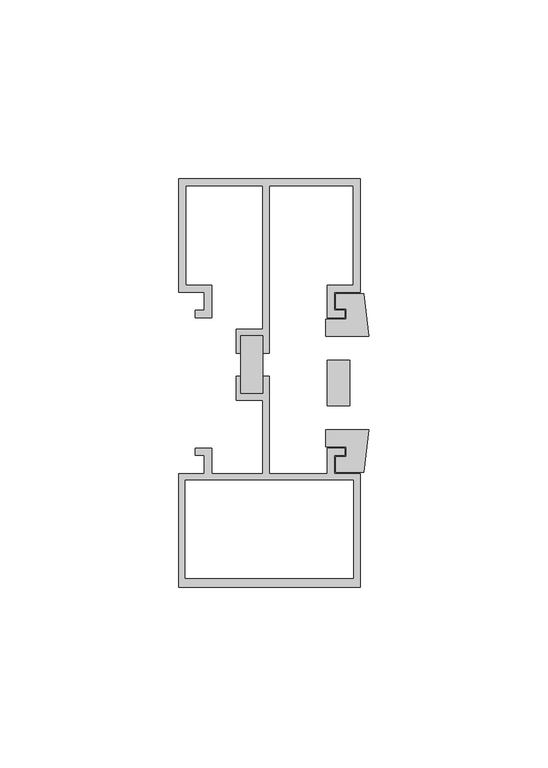
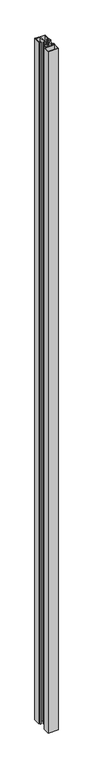
"""IFC4 building model written with IfcOpenShell, lengths in millimetres: proxy geometry, Generic Models 3:Generic Models 1:5:Generic Models 1:5 : Generic Models 3:Generic Models 1:300625:345888:Generic Models 1:5:Generic Models 1:5 : Generic Models 3:Generic Models 1:300625:345888 : Generic Models 3:Generic Models 1:5:Generic Models 1:5 : Generic Models 3:Generic Models 1:300625:345888:5 : Generic Models 3:Generic Models 1:5:Generic Models 1:5 : Generic Models 3:Generic Models 1:300625:345888:Generic Models 1:5:Generic Models 1:5 : Generic Models 3:Generic Models 1:300625:345888 : Generic Models 3:Generic Models 1:5:Generic Models 1:5 : Generic Models 3:Generic Models 1:300625:345888:301574."""

from ifc_helpers import new_model, si_unit, frame, origin, place, context, project, spatial, polyline, outline, extrude, source, transform, mapped, element, save


def generic_models_8cb2473c(model_context):
    return source(origin(), model_context, "Body", "SweptSolid", [
        extrude(outline(polyline([(592785.2574021, -579063.9802804), (592779.1776149, -579063.9802804), (592779.1776149, -579047.8688442), (592785.2574021, -579047.8688442), (592785.2574021, -579063.9802804)])), frame((0.0, 0.0, 66.3122056), z_axis=(0.0, 0.0, 1.0), x_axis=(1.0, 0.0, 0.0)), (0.0, 0.0, 1.0), 3584.971571),
        extrude(outline(polyline([(592809.6883176, -579067.3663841), (592803.3447692, -579067.3663841), (592803.3447692, -579054.6663841), (592809.6883176, -579054.6663841), (592809.6883176, -579067.3663841)])), frame((0.0, 0.0, 66.3122056), z_axis=(0.0, 0.0, 1.0), x_axis=(1.0, 0.0, 0.0)), (0.0, 0.0, 1.0), 3584.971571),
        extrude(outline(polyline([(592808.6614348, -579078.8588708), (592802.9478941, -579078.8588708), (592802.9478941, -579074.1048149), (592815.0181513, -579074.1048149), (592813.5572844, -579086.0026208), (592805.717575, -579086.0026208), (592805.717575, -579081.704549), (592808.6614348, -579081.704549), (592808.6614348, -579078.8588708)])), frame((0.0, 0.0, 66.3122056), z_axis=(0.0, 0.0, 1.0), x_axis=(1.0, 0.0, 0.0)), (0.0, 0.0, 1.0), 3584.971571),
        extrude(outline(polyline([(592813.5572844, -579036.0301474), (592815.0181513, -579047.9279532), (592802.9478941, -579047.9279532), (592802.9478941, -579043.1738974), (592808.6614348, -579043.1738974), (592808.6614348, -579040.3282192), (592805.717575, -579040.3282192), (592805.717575, -579036.0301474), (592813.5572844, -579036.0301474)])), frame((0.0, 0.0, 66.3122056), z_axis=(0.0, 0.0, 1.0), x_axis=(1.0, 0.0, 0.0)), (0.0, 0.0, 1.0), 3584.9377944),
        extrude(outline(polyline([(592761.7742239, -579118.1663841), (592761.7742239, -579086.3994958), (592768.9939713, -579086.3994958), (592768.9939713, -579081.307674), (592766.4747398, -579081.307674), (592766.4747398, -579079.2557458), (592771.0458995, -579079.2557458), (592771.0458995, -579086.3994958), (592785.2574021, -579086.3994958), (592785.2574021, -579065.8802139), (592777.8856601, -579065.8802139), (592777.8856601, -579059.1164506), (592779.1776149, -579059.1164506), (592779.1776149, -579063.9802804), (592785.2574021, -579063.9802804), (592785.2574021, -579059.1164506), (592787.1573356, -579059.1164506), (592787.1573356, -579086.3994958), (592803.3447691, -579086.3994958), (592803.3447691, -579079.2557458), (592808.2645598, -579079.2557458), (592808.2645598, -579081.307674), (592805.3207, -579081.307674), (592805.3207, -579086.3994958), (592812.5404473, -579086.3994958), (592812.5404473, -579118.1663841), (592761.7742239, -579118.1663841)]), holes=[polyline([(592810.6405138, -579088.2994293), (592763.6741574, -579088.2994293), (592763.6741574, -579115.6584719), (592810.6405138, -579115.6584719), (592810.6405138, -579088.2994293)])]), frame((0.0, 0.0, 66.3122056), z_axis=(0.0, 0.0, 1.0), x_axis=(1.0, 0.0, 0.0)), (0.0, 0.0, 1.0), 3584.971571),
        extrude(outline(polyline([(592808.2645598, -579040.7250942), (592808.2645598, -579042.7770224), (592803.3447691, -579042.7770224), (592803.3447691, -579033.7333389), (592810.6306483, -579033.7333389), (592810.6306483, -579005.8423149), (592787.1573356, -579005.8423149), (592787.1573356, -579052.732674), (592785.2574021, -579052.732674), (592785.2574021, -579047.8688442), (592779.1776149, -579047.8688442), (592779.1776149, -579052.732674), (592777.8856601, -579052.732674), (592777.8856601, -579045.9689107), (592785.2574021, -579045.9689107), (592785.2574021, -579005.8423149), (592763.6964365, -579005.8423149), (592763.6964365, -579033.7333389), (592771.0458995, -579033.7333389), (592771.0458995, -579042.7770224), (592766.4747398, -579042.7770224), (592766.4747398, -579040.7250942), (592768.9939713, -579040.7250942), (592768.9939713, -579035.6332724), (592761.7742239, -579035.6332724), (592761.7742239, -579003.8663841), (592812.5404473, -579003.8663841), (592812.5404473, -579035.6332724), (592805.3207, -579035.6332724), (592805.3207, -579040.7250942), (592808.2645598, -579040.7250942)])), frame((0.0, 0.0, 66.3122056), z_axis=(0.0, 0.0, 1.0), x_axis=(1.0, 0.0, 0.0)), (0.0, 0.0, 1.0), 3584.971571),
    ])


if __name__ == "__main__":
    model = new_model("IFC4")
    model_context = context("Model", 3, world=origin())
    ifc_project = project(units=[si_unit("LENGTHUNIT", "METRE", prefix="MILLI")], contexts=[model_context])
    site = spatial("IfcSite", under=ifc_project)
    building = spatial("IfcBuilding", under=site)
    placement = place(None, origin())
    generic_models_shape = generic_models_8cb2473c(model_context)
    element("IfcBuildingElementProxy", 1, Name="Generic Models 3:Generic Models 1:5:Generic Models 1:5 : Generic Models 3:Generic Models 1:300625:345888:Generic Models 1:5:Generic Models 1:5 : Generic Models 3:Generic Models 1:300625:345888 : Generic Models 3:Generic Models 1:5:Generic Models 1:5 : Generic Models 3:Generic Models 1:300625:345888:5 : Generic Models 3:Generic Models 1:5:Generic Models 1:5 : Generic Models 3:Generic Models 1:300625:345888:Generic Models 1:5:Generic Models 1:5 : Generic Models 3:Generic Models 1:300625:345888 : Generic Models 3:Generic Models 1:5:Generic Models 1:5 : Generic Models 3:Generic Models 1:300625:345888:301574", ObjectType="Generic Models 3:Generic Models 1:5:Generic Models 1:5 : Generic Models 3:Generic Models 1:300625:345888:Generic Models 1:5:Generic Models 1:5 : Generic Models 3:Generic Models 1:300625:345888 : Generic Models 3:Generic Models 1:5:Generic Models 1:5 : Generic Models 3:Generic Models 1:300625:345888:5 : Generic Models 3:Generic Models 1:5:Generic Models 1:5 : Generic Models 3:Generic Models 1:300625:345888:Generic Models 1:5:Generic Models 1:5 : Generic Models 3:Generic Models 1:300625:345888 : Generic Models 3:Generic Models 1:5:Generic Models 1:5 : Generic Models 3:Generic Models 1:300625:345888:301574", at=placement, inside=building, context=model_context, shape_type="MappedRepresentation", body=[
        mapped(generic_models_shape, transform((0.0, 0.0, 0.0), x_axis=(1.0, 0.0, 0.0), y_axis=(0.0, 1.0, 0.0), z_axis=(0.0, 0.0, 1.0))),
    ])
    save(model, "model.ifc")

# Revit data of these elements
# Type "Generic Models 3:Generic Models 1:5:Generic Models 1:5 : Generic Models 3:Generic Models 1:300625:345888:Generic Models 1:5:Generic Models 1:5 : Generic Models 3:Generic Models 1:300625:345888 : Generic Models 3:Generic Models 1:5:Generic Models 1:5 : Generic Models 3:Generic Models 1:300625:345888:5 : Generic Models 3:Generic Models 1:5:Generic Models 1:5 : Generic Models 3:Generic Models 1:300625:345888:Generic Models 1:5:Generic Models 1:5 : Generic Models 3:Generic Models 1:300625:345888 : Generic Models 3:Generic Models 1:5:Generic Models 1:5 : Generic Models 3:Generic Models 1:300625:345888:301574"
#   NameOverride = "Generic Models 3:Generic Models 1:5:Generic Models 1:5 : Generic Models 3:Generic Models 1:300625:345888:Generic Models 1:5:Generic Models 1:5 : Generic Models 3:Generic Models 1:300625:345888 : Generic Models 3:Generic Models 1:5:Generic Models 1:5 : Generic Models 3:Generic Models 1:300625:345888:301574"
#   ObjectTypeOverride = "Generic Models 1:5:Generic Models 1:5 : Generic Models 3:Generic Models 1:300625:345888 : Generic Models 3:Generic Models 1:5:Generic Models 1:5 : Generic Models 3:Generic Models 1:300625:345888"
#   Reference = "Generic Models 1"
#   Tag = "301574"
# Element 1 (IfcBuildingElementProxy, "Generic Models 3:Generic Models 1:5:Generic Models 1:5 : Generic Models 3:Generic Models 1:300625:345888:Generic Models 1:5:Generic Models 1:5 : Generic Models 3:Generic Models 1:300625:345888 : Generic Models 3:Generic Models 1:5:Generic Models 1:5 : Generic Models 3:Generic Models 1:300625:345888:5 : Generic Models 3:Generic Models 1:5:Generic Models 1:5 : Generic Models 3:Generic Models 1:300625:345888:Generic Models 1:5:Generic Models 1:5 : Generic Models 3:Generic Models 1:300625:345888 : Generic Models 3:Generic Models 1:5:Generic Models 1:5 : Generic Models 3:Generic Models 1:300625:345888:301574")
#   Materials on its faces: "THERMAL BROKEN ALUMINUM STOREFRONT"
# Materials
#   "THERMAL BROKEN ALUMINUM STOREFRONT": class "Unassigned", colour RGB 244 244 244, transparency 0, Cost = 0
